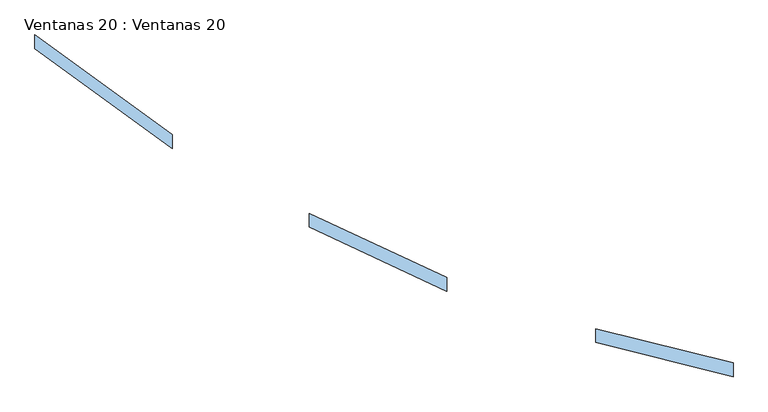
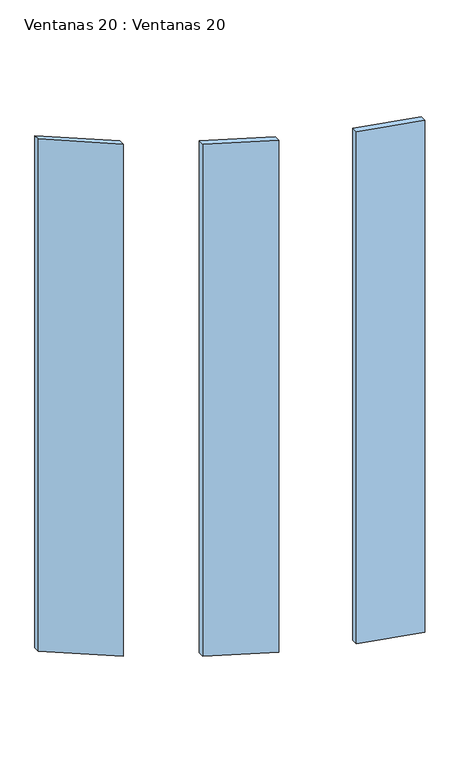
"""IFC4 building model written with IfcOpenShell, lengths in millimetres: window geometry, Ventanas 20 : Ventanas 20."""

from ifc_helpers import new_model, si_unit, frame, origin, place, context, project, spatial, polyline, outline, extrude, source, transform, mapped, element, save


def ventanas_20_ventanas_20_f7ffd275(model_context):
    return source(origin(), model_context, "Body", "SweptSolid", [
        extrude(outline(polyline([(-10381.5702783, 6129.993821), (-10381.5702783, 6109.993821), (-10581.5702783, 6255.3023266), (-10581.5702783, 6275.3023266), (-10381.5702783, 6129.993821)])), frame((0.0, 0.0, 6283.3221536), z_axis=(0.0, 0.0, 1.0), x_axis=(1.0, 0.0, 0.0)), (0.0, 0.0, 1.0), 1809.3949991),
        extrude(outline(polyline([(-9982.794852, 5921.9692435), (-9982.794852, 5901.9692435), (-10182.794852, 5995.2307751), (-10182.794852, 6015.2307751), (-9982.794852, 5921.9692435)])), frame((0.0, 0.0, 6283.3221536), z_axis=(0.0, 0.0, 1.0), x_axis=(1.0, 0.0, 0.0)), (0.0, 0.0, 1.0), 1809.3949991),
        extrude(outline(polyline([(-9565.89327, 5797.4184388), (-9565.89327, 5777.4184388), (-9765.89327, 5827.2840394), (-9765.89327, 5847.2840394), (-9565.89327, 5797.4184388)])), frame((0.0, 0.0, 6283.3221536), z_axis=(0.0, 0.0, 1.0), x_axis=(1.0, 0.0, 0.0)), (0.0, 0.0, 1.0), 1809.3949991),
    ])


if __name__ == "__main__":
    model = new_model("IFC4")
    model_context = context("Model", 3, world=origin())
    ifc_project = project(units=[si_unit("LENGTHUNIT", "METRE", prefix="MILLI")], contexts=[model_context])
    site = spatial("IfcSite", under=ifc_project)
    building = spatial("IfcBuilding", under=site)
    placement = place(None, origin())
    ventanas_20_ventanas_20_shape = ventanas_20_ventanas_20_f7ffd275(model_context)
    element("IfcWindow", 1, ObjectType="Ventanas 20 : Ventanas 20", at=placement, inside=building, context=model_context, shape_type="MappedRepresentation", body=[
        mapped(ventanas_20_ventanas_20_shape, transform((0.0, 0.0, 0.0), x_axis=(1.0, 0.0, 0.0), y_axis=(0.0, 1.0, 0.0), z_axis=(0.0, 0.0, 1.0))),
    ])
    save(model, "model.ifc")

# Revit data of these elements
# Type "Ventanas 20 : Ventanas 20"
#   Type Mark = "46"
# Element 1 (IfcWindow, "Ventanas 20 : Ventanas 20")
#   Materials on its faces: "VIDRIO"
# Materials
#   "VIDRIO": class "Genérico", colour RGB 120 120 120, transparency 0, Cost = 0
